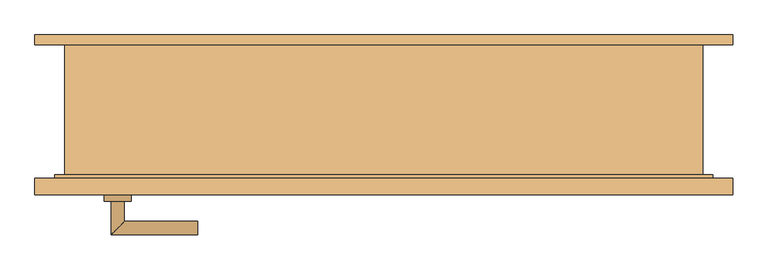
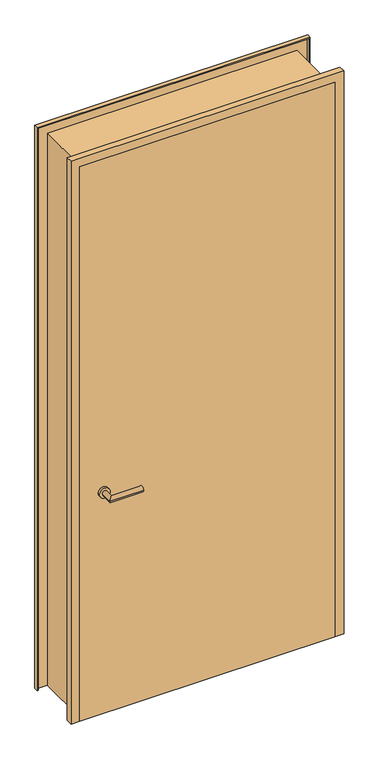
"""IFC4 building model written with IfcOpenShell, lengths in millimetres: door geometry, Drehflügel 1-flg - Variabel : Drehflügel 1-flg - Variabel."""

from ifc_helpers import new_model, si_unit, point, frame, frame_2d, origin, origin_with_axes, place, context, project, spatial, polyline, circle_curve, ellipse_curve, trimmed, segment, composite_curve, outline, extrude, faceted_brep, source, transform, mapped, element, save
from ifc_brep_helpers import plane_surface, cylinder_surface, advanced_brep


def door_730112ad(model_context):
    return source(origin(), model_context, "Body", "SolidModel", [
        advanced_brep(
        [(-410.0, -89.4346141, 900.0), (-390.0, -89.4346141, 900.0), (-390.0, -39.4346141, 900.0), (-410.0, -19.4346141, 900.0), (-280.0, -19.4346141, 900.0), (-280.0, -39.4346141, 900.0)],
        [
            (0, 1, circle_curve(frame((-400.0, -89.4346141, 900.0), z_axis=(0.0, -1.0, 0.0), x_axis=(1.0, 0.0, 0.0)), 10.0)),
            (1, 0, circle_curve(frame((-400.0, -89.4346141, 900.0), z_axis=(0.0, -1.0, 0.0), x_axis=(1.0, 0.0, 0.0)), 10.0)),
            (1, 2),
            (2, 3, ellipse_curve(frame((-400.0, -29.4346141, 900.0), z_axis=(-0.7071067811865385, -0.7071067811865565, 0.0), x_axis=(0.7071067811865563, -0.7071067811865386, 0.0)), 14.1421356, 10.0)),
            (3, 0),
            (3, 2, ellipse_curve(frame((-400.0, -29.4346141, 900.0), z_axis=(-0.7071067811865385, -0.7071067811865565, 0.0), x_axis=(0.7071067811865563, -0.7071067811865386, 0.0)), 14.1421356, 10.0)),
            (4, 5, circle_curve(frame((-280.0, -29.4346141, 900.0), z_axis=(1.0, 0.0, 0.0), x_axis=(0.0, -1.0, 0.0)), 10.0)),
            (5, 4, circle_curve(frame((-280.0, -29.4346141, 900.0), z_axis=(1.0, 0.0, 0.0), x_axis=(0.0, -1.0, 0.0)), 10.0)),
            (2, 5),
            (4, 3),
        ],
        [
            plane_surface(frame((-400.0, -89.4346141, -387.7526403), z_axis=(0.0, -1.0, 0.0), x_axis=(0.0, 0.0, 1.0))),
            cylinder_surface(frame((-400.0, -89.4346141, 900.0), z_axis=(0.0, -1.0, 0.0), x_axis=(1.0, 0.0, 0.0)), 10.0),
            plane_surface(frame((-280.0, -29.4346141, -387.7526403), z_axis=(1.0, 0.0, 0.0), x_axis=(0.0, 0.0, 1.0))),
            cylinder_surface(frame((-400.0, -29.4346141, 900.0), z_axis=(-1.0, 0.0, 0.0), x_axis=(0.0, -1.0, 0.0)), 10.0),
        ],
        [
            (0, [[1, 2]]),
            (1, [[3, 4, 5, -2]]),
            (1, [[-5, 6, -3, -1]]),
            (2, [[7, 8]]),
            (3, [[9, -7, 10, -4]]),
            (3, [[-10, -8, -9, -6]]),
        ],
    ),
        advanced_brep(
        [(-390.0, -149.4346141, 900.0), (-410.0, -149.4346141, 900.0), (-410.0, -199.4346141, 900.0), (-390.0, -179.4346141, 900.0), (-280.0, -179.4346141, 900.0), (-280.0, -199.4346141, 900.0)],
        [
            (0, 1, circle_curve(frame((-400.0, -149.4346141, 900.0), z_axis=(0.0, 1.0, 0.0), x_axis=(-1.0, 0.0, 0.0)), 10.0)),
            (1, 0, circle_curve(frame((-400.0, -149.4346141, 900.0), z_axis=(0.0, 1.0, 0.0), x_axis=(-1.0, 0.0, 0.0)), 10.0)),
            (1, 2),
            (2, 3, ellipse_curve(frame((-400.0, -189.4346141, 900.0), z_axis=(-0.7071067811865475, 0.7071067811865475, 0.0), x_axis=(0.7071067811865474, 0.7071067811865476, 0.0)), 14.1421356, 10.0)),
            (3, 0),
            (3, 2, ellipse_curve(frame((-400.0, -189.4346141, 900.0), z_axis=(-0.7071067811865475, 0.7071067811865475, 0.0), x_axis=(0.7071067811865474, 0.7071067811865476, 0.0)), 14.1421356, 10.0)),
            (4, 5, circle_curve(frame((-280.0, -189.4346141, 900.0), z_axis=(1.0, 0.0, 0.0), x_axis=(0.0, -1.0, 0.0)), 10.0)),
            (5, 4, circle_curve(frame((-280.0, -189.4346141, 900.0), z_axis=(1.0, 0.0, 0.0), x_axis=(0.0, -1.0, 0.0)), 10.0)),
            (2, 5),
            (4, 3),
        ],
        [
            plane_surface(frame((-400.0, -149.4346141, -387.7526403), z_axis=(0.0, 1.0, 0.0), x_axis=(0.0, 0.0, 1.0))),
            cylinder_surface(frame((-400.0, -149.4346141, 900.0), z_axis=(0.0, 1.0, 0.0), x_axis=(-1.0, 0.0, 0.0)), 10.0),
            plane_surface(frame((-280.0, -189.4346141, -387.7526403), z_axis=(1.0, 0.0, 0.0), x_axis=(0.0, 0.0, 1.0))),
            cylinder_surface(frame((-400.0, -189.4346141, 900.0), z_axis=(-1.0, 0.0, 0.0), x_axis=(0.0, -1.0, 0.0)), 10.0),
        ],
        [
            (0, [[1, 2]]),
            (1, [[3, 4, 5, -2]]),
            (1, [[-5, 6, -3, -1]]),
            (2, [[7, 8]]),
            (3, [[9, -7, 10, -4]]),
            (3, [[-10, -8, -9, -6]]),
        ],
    ),
        extrude(outline(composite_curve([segment(trimmed(circle_curve(frame_2d((900.0, -400.0)), 20.0), [point((900.0, -420.0))], [point((900.0, -380.0))], False, "CARTESIAN"), True, "CONTINUOUS"), segment(trimmed(circle_curve(frame_2d((900.0, -400.0)), 20.0), [point((900.0, -380.0))], [point((900.0, -420.0))], False, "CARTESIAN"), True, "CONTINUOUS")], self_intersect=False)), frame((0.0, -89.4346141, 0.0), z_axis=(0.0, 1.0, 0.0), x_axis=(0.0, 0.0, 1.0)), (0.0, 0.0, 1.0), 10.0),
        extrude(outline(composite_curve([segment(trimmed(circle_curve(frame_2d((900.0, -400.0)), 20.0), [point((900.0, -420.0))], [point((900.0, -380.0))], False, "CARTESIAN"), True, "CONTINUOUS"), segment(trimmed(circle_curve(frame_2d((900.0, -400.0)), 20.0), [point((900.0, -380.0))], [point((900.0, -420.0))], False, "CARTESIAN"), True, "CONTINUOUS")], self_intersect=False)), frame((0.0, -149.4346141, 0.0), z_axis=(0.0, 1.0, 0.0), x_axis=(0.0, 0.0, 1.0)), (0.0, 0.0, 1.0), 10.0),
        extrude(outline(polyline([(490.0, -114.4346141), (490.0, -139.4346141), (-490.0, -139.4346141), (-490.0, -114.4346141), (490.0, -114.4346141)])), origin_with_axes(), (0.0, 0.0, 1.0), 2250.0),
        faceted_brep([(524.4603207, 100.5653859, 0.0), (524.4603207, 85.5653859, 0.0), (519.4603207, 85.5653859, 0.0), (519.4603207, 95.5653859, 0.0), (480.0, 95.5653859, 0.0), (480.0, -109.4346141, 0.0), (495.0, -109.4346141, 0.0), (495.0, -134.4346141, 0.0), (519.4603207, -134.4346141, 0.0), (519.4603207, -114.4346141, 0.0), (524.4603207, -114.4346141, 0.0), (524.4603207, -139.4346141, 0.0), (490.0, -139.4346141, 0.0), (490.0, -114.4346141, 0.0), (475.0, -114.4346141, 0.0), (475.0, 100.5653859, 0.0), (475.0, 100.5653859, 2235.0), (-475.0, 100.5653859, 2235.0), (-475.0, 100.5653859, 0.0), (-524.4603207, 100.5653859, 0.0), (-524.4603207, 100.5653859, 2284.4603207), (524.4603207, 100.5653859, 2284.4603207), (475.0, -114.4346141, 2235.0), (490.0, -114.4346141, 2250.0), (-490.0, -114.4346141, 2250.0), (-490.0, -114.4346141, 0.0), (-475.0, -114.4346141, 0.0), (-475.0, -114.4346141, 2235.0), (490.0, -139.4346141, 2250.0), (524.4603207, -139.4346141, 2284.4603207), (-524.4603207, -139.4346141, 2284.4603207), (-524.4603207, -139.4346141, 0.0), (-490.0, -139.4346141, 0.0), (-490.0, -139.4346141, 2250.0), (524.4603207, -114.4346141, 2284.4603207), (519.4603207, -114.4346141, 2279.4603207), (-519.4603207, -114.4346141, 2279.4603207), (-519.4603207, -114.4346141, 0.0), (-524.4603207, -114.4346141, 0.0), (-524.4603207, -114.4346141, 2284.4603207), (519.4603207, -134.4346141, 2279.4603207), (495.0, -134.4346141, 2255.0), (-495.0, -134.4346141, 2255.0), (-495.0, -134.4346141, 0.0), (-519.4603207, -134.4346141, 0.0), (-519.4603207, -134.4346141, 2279.4603207), (495.0, -109.4346141, 2255.0), (480.0, -109.4346141, 2240.0), (-480.0, -109.4346141, 2240.0), (-480.0, -109.4346141, 0.0), (-495.0, -109.4346141, 0.0), (-495.0, -109.4346141, 2255.0), (480.0, 95.5653859, 2240.0), (519.4603207, 95.5653859, 2279.4603207), (-519.4603207, 95.5653859, 2279.4603207), (-519.4603207, 95.5653859, 0.0), (-480.0, 95.5653859, 0.0), (-480.0, 95.5653859, 2240.0), (519.4603207, 85.5653859, 2279.4603207), (524.4603207, 85.5653859, 2284.4603207), (-524.4603207, 85.5653859, 2284.4603207), (-524.4603207, 85.5653859, 0.0), (-519.4603207, 85.5653859, 0.0), (-519.4603207, 85.5653859, 2279.4603207)], [[[0, 1, 2, 3, 4, 5, 6, 7, 8, 9, 10, 11, 12, 13, 14, 15]], [[15, 16, 17, 18, 19, 20, 21, 0]], [[14, 22, 16, 15]], [[13, 23, 24, 25, 26, 27, 22, 14]], [[12, 28, 23, 13]], [[11, 29, 30, 31, 32, 33, 28, 12]], [[10, 34, 29, 11]], [[9, 35, 36, 37, 38, 39, 34, 10]], [[8, 40, 35, 9]], [[7, 41, 42, 43, 44, 45, 40, 8]], [[6, 46, 41, 7]], [[5, 47, 48, 49, 50, 51, 46, 6]], [[4, 52, 47, 5]], [[3, 53, 54, 55, 56, 57, 52, 4]], [[2, 58, 53, 3]], [[1, 59, 60, 61, 62, 63, 58, 2]], [[0, 21, 59, 1]], [[20, 19, 61, 60]], [[19, 18, 26, 25, 32, 31, 38, 37, 44, 43, 50, 49, 56, 55, 62, 61]], [[27, 26, 18, 17]], [[33, 32, 25, 24]], [[39, 38, 31, 30]], [[45, 44, 37, 36]], [[51, 50, 43, 42]], [[57, 56, 49, 48]], [[63, 62, 55, 54]], [[22, 27, 17, 16]], [[28, 33, 24, 23]], [[34, 39, 30, 29]], [[40, 45, 36, 35]], [[46, 51, 42, 41]], [[52, 57, 48, 47]], [[58, 63, 54, 53]], [[21, 20, 60, 59]]]),
    ])


if __name__ == "__main__":
    model = new_model("IFC4")
    model_context = context("Model", 3, world=origin())
    ifc_project = project(units=[si_unit("LENGTHUNIT", "METRE", prefix="MILLI")], contexts=[model_context])
    site = spatial("IfcSite", under=ifc_project)
    building = spatial("IfcBuilding", under=site)
    placement = place(None, origin())
    door_shape = door_730112ad(model_context)
    element("IfcDoor", 1, ObjectType="Drehflügel 1-flg - Variabel : Drehflügel 1-flg - Variabel", at=placement, inside=building, context=model_context, shape_type="MappedRepresentation", body=[
        mapped(door_shape, transform((0.0, 0.0, 0.0), x_axis=(1.0, 0.0, 0.0), y_axis=(0.0, 1.0, 0.0), z_axis=(0.0, 0.0, 1.0))),
    ])
    save(model, "model.ifc")

# Revit data of these elements
# Type "Drehflügel 1-flg - Variabel : Drehflügel 1-flg - Variabel"
#   Construction Type Id = "MDOOR"
#   Type Mark = "15"
#   Operation = "SingleSwingRight"
#   Keynote = "16.03"
#   Analytic Construction = "Metall"
#   Thermal Resistance (R) = 0.270117 (m²·K)/W
#   Heat Transfer Coefficient (U) = 3.7021 W/(m²·K)
#   Rough Width [instance default] = 1.000 m
#   Rough Height [instance default] = 2.360 m
#   Höhe Türgriff [instance default] = 0.900 m
#   Height [instance default] = 2.260 m
#   Fußbodenaufbau [instance default] = 0.100 m
#   Width [instance default] = 1.000 m
#   Sichtbarkeit Sturzlinien [instance default] = yes
#   Türgriff auswählen [instance default] = element 217699
#   Türgriff [instance default] = none
#   Türflügel [instance default] = none
#   Rahmen/Pfosten [instance default] = Metall - Lackiert - Grau
#   Visual Light Transmittance = 0
#   Solar Heat Gain Coefficient = 0
#   Function = (empty or 0)
#   Wall Closure = (empty or 0)
# Element 1 (IfcDoor, "Drehflügel 1-flg - Variabel : Drehflügel 1-flg - Variabel")
#   Rough Height = 2.260 m
#   Fußbodenaufbau = 0.000 m
#   Materials on its faces: "Metall - Lackiert - Grau", "Metall - Chrom", "Holz - Birke"
# Materials
#   "Metall - Lackiert - Grau": class "Farbe 1", colour RGB 98 98 98, transparency 0, Cost = 0
#   "Metall - Chrom": class "Metall", colour RGB 247 247 247, transparency 0, Cost = 0
#   "Holz - Birke": class "Holz", colour RGB 213 164 103, transparency 0, Cost = 0
